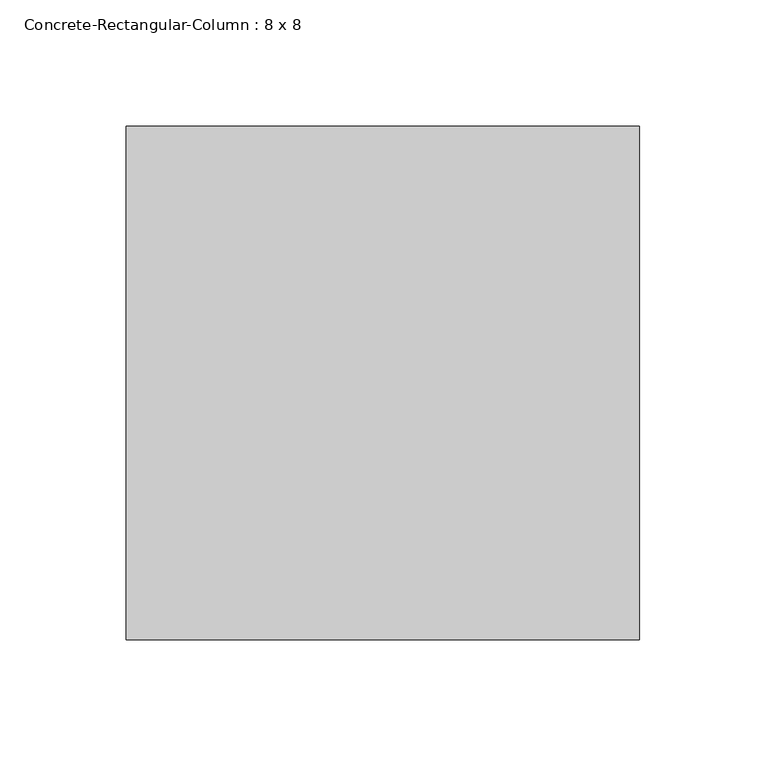
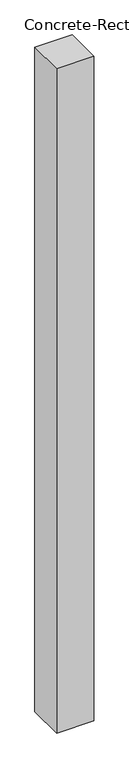
"""IFC4 building model written with IfcOpenShell, lengths in millimetres: column geometry, Concrete-Rectangular-Column : 8 x 8."""

from ifc_helpers import new_model, si_unit, origin, origin_with_axes, place, context, project, spatial, polyline, outline, extrude, source, transform, mapped, element, save


def concrete_rectangular_column_8_x_8_cc1d8254(model_context):
    return source(origin(), model_context, "Body", "SweptSolid", [
        extrude(outline(polyline([(101.6, -101.6), (-101.6, -101.6), (-101.6, 101.6), (101.6, 101.6), (101.6, -101.6)])), origin_with_axes(), (0.0, 0.0, 1.0), 3810.0),
    ])


if __name__ == "__main__":
    model = new_model("IFC4")
    model_context = context("Model", 3, world=origin())
    ifc_project = project(units=[si_unit("LENGTHUNIT", "METRE", prefix="MILLI")], contexts=[model_context])
    site = spatial("IfcSite", under=ifc_project)
    building = spatial("IfcBuilding", under=site)
    placement = place(None, origin())
    concrete_rectangular_column_8_x_8_shape = concrete_rectangular_column_8_x_8_cc1d8254(model_context)
    element("IfcColumn", 1, ObjectType="Concrete-Rectangular-Column : 8 x 8", at=placement, inside=building, context=model_context, shape_type="MappedRepresentation", body=[
        mapped(concrete_rectangular_column_8_x_8_shape, transform((0.0, 0.0, 0.0), x_axis=(1.0, 0.0, 0.0), y_axis=(0.0, 1.0, 0.0), z_axis=(0.0, 0.0, 1.0))),
    ])
    save(model, "model.ifc")

# Revit data of these elements
# Type "Concrete-Rectangular-Column : 8 x 8"
#   Assembly Code = "B10"
#   b = 203.2 mm
#   h = 203.2 mm
#   Structural Material [instance default] = Concrete - Cast-in-Place Concrete
# Element 1 (IfcColumn, "Concrete-Rectangular-Column : 8 x 8")
#   Materials on its faces: "Concrete - Cast-in-Place Concrete"
# Materials
#   "Concrete - Cast-in-Place Concrete": class "Concrete", colour RGB 192 192 192, transparency 0
